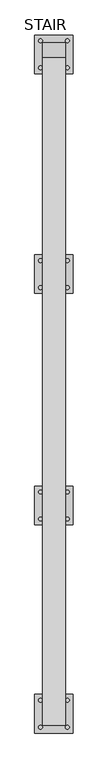
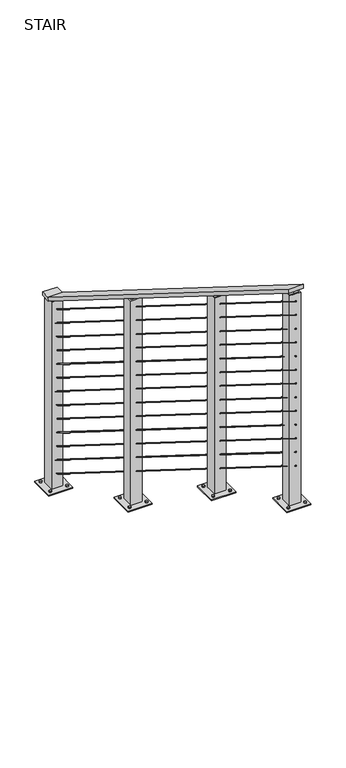
"""IFC4 building model written with IfcOpenShell, lengths in millimetres: railing geometry, STAIR."""

from ifc_helpers import new_model, si_unit, point, frame, frame_2d, origin, origin_with_axes, place, context, project, spatial, polyline, circle_curve, ellipse_curve, trimmed, segment, composite_curve, outline, extrude, faceted_brep, source, transform, mapped, element, save
from ifc_brep_helpers import plane_surface, cylinder_surface, advanced_brep


def stair_e71d8709(model_context):
    return source(origin(), model_context, "Body", "SolidModel", [
        faceted_brep([(27258.1620052, 6154.2043237, 1066.8), (27334.3620052, 6154.2043237, 1066.8), (27334.3620052, 6154.2043237, 1047.75), (27258.1620052, 6154.2043237, 1047.75), (27258.1620052, 6106.1413199, 1066.8), (27334.3620052, 6106.1413199, 1066.8), (27334.3620052, 6100.6673274, 1047.75), (27258.1620052, 3906.3043237, 2444.8228911), (27258.1620052, 3906.3043237, 2422.3438702), (27334.3620052, 3906.3043237, 2422.3438702), (27334.3620052, 3906.3043237, 2444.8228911), (27258.1620052, 6100.6673274, 1047.75)], [[[0, 1, 2, 3]], [[1, 0, 4, 5]], [[2, 1, 5, 6]], [[7, 8, 9, 10]], [[5, 4, 7, 10]], [[6, 5, 10, 9]], [[3, 2, 6, 11]], [[0, 3, 11, 4]], [[11, 6, 9, 8]], [[4, 11, 8, 7]]]),
        advanced_brep(
        [(27298.6432552, 6154.2043237, 988.21875), (27293.8807552, 6154.2043237, 988.21875), (27298.6432552, 3906.3043237, 2364.0985031), (27293.8807552, 3906.3043237, 2364.0985031), (27298.6432552, 6102.7200746, 988.21875), (27293.8807552, 6102.7200746, 988.21875)],
        [
            (0, 1, circle_curve(frame((27296.2620052, 6154.2043237, 988.21875), z_axis=(0.0, 1.0, 0.0), x_axis=(-1.0, 0.0, 0.0)), 2.38125)),
            (1, 0, circle_curve(frame((27296.2620052, 6154.2043237, 988.21875), z_axis=(0.0, 1.0, 0.0), x_axis=(-1.0, 0.0, 0.0)), 2.38125)),
            (2, 3, ellipse_curve(frame((27296.2620052, 3906.3043237, 2364.0985031), z_axis=(0.0, -1.0, 0.0), x_axis=(0.0, 0.0, -1.0)), 2.8098776, 2.38125)),
            (3, 2, ellipse_curve(frame((27296.2620052, 3906.3043237, 2364.0985031), z_axis=(0.0, -1.0, 0.0), x_axis=(0.0, 0.0, -1.0)), 2.8098776, 2.38125)),
            (0, 4),
            (4, 5, ellipse_curve(frame((27296.2620052, 6102.7200746, 988.21875), z_axis=(0.0, 0.9611079128273463, -0.2761730977134851), x_axis=(0.0, 0.27617309771348497, 0.9611079128273464)), 2.4776094, 2.38125)),
            (5, 1),
            (5, 4, ellipse_curve(frame((27296.2620052, 6102.7200746, 988.21875), z_axis=(0.0, 0.9611079128273463, -0.2761730977134851), x_axis=(0.0, 0.27617309771348497, 0.9611079128273464)), 2.4776094, 2.38125)),
            (4, 2),
            (3, 5),
        ],
        [
            plane_surface(frame((27296.2620052, 6154.2043237, 990.6), z_axis=(0.0, 1.0, 0.0), x_axis=(0.0, 0.0, -1.0))),
            plane_surface(frame((27296.2620052, 3906.3043237, 2366.9083807), z_axis=(0.0, -1.0, 0.0), x_axis=(0.0, 0.0, -1.0))),
            cylinder_surface(frame((27296.2620052, 6154.2043237, 988.21875), z_axis=(0.0, 1.0, 0.0), x_axis=(-1.0, 0.0, 0.0)), 2.38125),
            cylinder_surface(frame((27296.2620052, 6102.1402031, 988.5819934), z_axis=(0.0, 0.8474568401986756, -0.5308642990449408), x_axis=(-1.0, 0.0, 0.0)), 2.38125),
        ],
        [
            (0, [[1, 2]]),
            (1, [[3, 4]]),
            (2, [[-1, 5, 6, 7]]),
            (2, [[-2, -7, 8, -5]]),
            (3, [[-6, 9, -4, 10]]),
            (3, [[-8, -10, -3, -9]]),
        ],
    ),
        advanced_brep(
        [(27298.6432552, 6154.2043237, 912.01875), (27293.8807552, 6154.2043237, 912.01875), (27298.6432552, 6102.7200746, 912.01875), (27293.8807552, 6102.7200746, 912.01875), (27298.6432552, 3906.3043237, 2287.8985031), (27293.8807552, 3906.3043237, 2287.8985031)],
        [
            (0, 1, circle_curve(frame((27296.2620052, 6154.2043237, 912.01875), z_axis=(0.0, 1.0, 0.0), x_axis=(-1.0, 0.0, 0.0)), 2.38125)),
            (1, 0, circle_curve(frame((27296.2620052, 6154.2043237, 912.01875), z_axis=(0.0, 1.0, 0.0), x_axis=(-1.0, 0.0, 0.0)), 2.38125)),
            (0, 2),
            (2, 3, ellipse_curve(frame((27296.2620052, 6102.7200746, 912.01875), z_axis=(0.0, 0.9611079128273463, -0.2761730977134851), x_axis=(0.0, 0.27617309771348497, 0.9611079128273464)), 2.4776094, 2.38125)),
            (3, 1),
            (3, 2, ellipse_curve(frame((27296.2620052, 6102.7200746, 912.01875), z_axis=(0.0, 0.9611079128273463, -0.2761730977134851), x_axis=(0.0, 0.27617309771348497, 0.9611079128273464)), 2.4776094, 2.38125)),
            (4, 5, ellipse_curve(frame((27296.2620052, 3906.3043237, 2287.8985031), z_axis=(0.0, -1.0, 0.0), x_axis=(0.0, 0.0, -1.0)), 2.8098776, 2.38125)),
            (5, 4, ellipse_curve(frame((27296.2620052, 3906.3043237, 2287.8985031), z_axis=(0.0, -1.0, 0.0), x_axis=(0.0, 0.0, -1.0)), 2.8098776, 2.38125)),
            (2, 4),
            (5, 3),
        ],
        [
            plane_surface(frame((27296.2620052, 6154.2043237, 914.4), z_axis=(0.0, 1.0, 0.0), x_axis=(0.0, 0.0, -1.0))),
            cylinder_surface(frame((27296.2620052, 6154.2043237, 912.01875), z_axis=(0.0, 1.0, 0.0), x_axis=(-1.0, 0.0, 0.0)), 2.38125),
            plane_surface(frame((27296.2620052, 3906.3043237, 2290.7083807), z_axis=(0.0, -1.0, 0.0), x_axis=(0.0, 0.0, -1.0))),
            cylinder_surface(frame((27296.2620052, 6102.1402031, 912.3819934), z_axis=(0.0, 0.8474568401986756, -0.5308642990449408), x_axis=(-1.0, 0.0, 0.0)), 2.38125),
        ],
        [
            (0, [[1, 2]]),
            (1, [[-1, 3, 4, 5]]),
            (1, [[-2, -5, 6, -3]]),
            (2, [[7, 8]]),
            (3, [[-4, 9, -8, 10]]),
            (3, [[-6, -10, -7, -9]]),
        ],
    ),
        advanced_brep(
        [(27298.6432552, 6154.2043237, 835.81875), (27293.8807552, 6154.2043237, 835.81875), (27298.6432552, 6102.7200746, 835.81875), (27293.8807552, 6102.7200746, 835.81875), (27298.6432552, 3906.3043237, 2211.6985031), (27293.8807552, 3906.3043237, 2211.6985031)],
        [
            (0, 1, circle_curve(frame((27296.2620052, 6154.2043237, 835.81875), z_axis=(0.0, 1.0, 0.0), x_axis=(-1.0, 0.0, 0.0)), 2.38125)),
            (1, 0, circle_curve(frame((27296.2620052, 6154.2043237, 835.81875), z_axis=(0.0, 1.0, 0.0), x_axis=(-1.0, 0.0, 0.0)), 2.38125)),
            (0, 2),
            (2, 3, ellipse_curve(frame((27296.2620052, 6102.7200746, 835.81875), z_axis=(0.0, 0.9611079128273463, -0.2761730977134851), x_axis=(0.0, 0.27617309771348497, 0.9611079128273464)), 2.4776094, 2.38125)),
            (3, 1),
            (3, 2, ellipse_curve(frame((27296.2620052, 6102.7200746, 835.81875), z_axis=(0.0, 0.9611079128273463, -0.2761730977134851), x_axis=(0.0, 0.27617309771348497, 0.9611079128273464)), 2.4776094, 2.38125)),
            (4, 5, ellipse_curve(frame((27296.2620052, 3906.3043237, 2211.6985031), z_axis=(0.0, -1.0, 0.0), x_axis=(0.0, 0.0, -1.0)), 2.8098776, 2.38125)),
            (5, 4, ellipse_curve(frame((27296.2620052, 3906.3043237, 2211.6985031), z_axis=(0.0, -1.0, 0.0), x_axis=(0.0, 0.0, -1.0)), 2.8098776, 2.38125)),
            (2, 4),
            (5, 3),
        ],
        [
            plane_surface(frame((27296.2620052, 6154.2043237, 838.2), z_axis=(0.0, 1.0, 0.0), x_axis=(0.0, 0.0, -1.0))),
            cylinder_surface(frame((27296.2620052, 6154.2043237, 835.81875), z_axis=(0.0, 1.0, 0.0), x_axis=(-1.0, 0.0, 0.0)), 2.38125),
            plane_surface(frame((27296.2620052, 3906.3043237, 2214.5083807), z_axis=(0.0, -1.0, 0.0), x_axis=(0.0, 0.0, -1.0))),
            cylinder_surface(frame((27296.2620052, 6102.1402031, 836.1819934), z_axis=(0.0, 0.8474568401986756, -0.5308642990449408), x_axis=(-1.0, 0.0, 0.0)), 2.38125),
        ],
        [
            (0, [[1, 2]]),
            (1, [[-1, 3, 4, 5]]),
            (1, [[-2, -5, 6, -3]]),
            (2, [[7, 8]]),
            (3, [[-4, 9, -8, 10]]),
            (3, [[-6, -10, -7, -9]]),
        ],
    ),
        advanced_brep(
        [(27298.6432552, 6154.2043237, 759.61875), (27293.8807552, 6154.2043237, 759.61875), (27298.6432552, 6102.7200746, 759.61875), (27293.8807552, 6102.7200746, 759.61875), (27298.6432552, 3906.3043237, 2135.4985031), (27293.8807552, 3906.3043237, 2135.4985031)],
        [
            (0, 1, circle_curve(frame((27296.2620052, 6154.2043237, 759.61875), z_axis=(0.0, 1.0, 0.0), x_axis=(-1.0, 0.0, 0.0)), 2.38125)),
            (1, 0, circle_curve(frame((27296.2620052, 6154.2043237, 759.61875), z_axis=(0.0, 1.0, 0.0), x_axis=(-1.0, 0.0, 0.0)), 2.38125)),
            (0, 2),
            (2, 3, ellipse_curve(frame((27296.2620052, 6102.7200746, 759.61875), z_axis=(0.0, 0.9611079128273463, -0.2761730977134851), x_axis=(0.0, 0.27617309771348497, 0.9611079128273464)), 2.4776094, 2.38125)),
            (3, 1),
            (3, 2, ellipse_curve(frame((27296.2620052, 6102.7200746, 759.61875), z_axis=(0.0, 0.9611079128273463, -0.2761730977134851), x_axis=(0.0, 0.27617309771348497, 0.9611079128273464)), 2.4776094, 2.38125)),
            (4, 5, ellipse_curve(frame((27296.2620052, 3906.3043237, 2135.4985031), z_axis=(0.0, -1.0, 0.0), x_axis=(0.0, 0.0, -1.0)), 2.8098776, 2.38125)),
            (5, 4, ellipse_curve(frame((27296.2620052, 3906.3043237, 2135.4985031), z_axis=(0.0, -1.0, 0.0), x_axis=(0.0, 0.0, -1.0)), 2.8098776, 2.38125)),
            (2, 4),
            (5, 3),
        ],
        [
            plane_surface(frame((27296.2620052, 6154.2043237, 762.0), z_axis=(0.0, 1.0, 0.0), x_axis=(0.0, 0.0, -1.0))),
            cylinder_surface(frame((27296.2620052, 6154.2043237, 759.61875), z_axis=(0.0, 1.0, 0.0), x_axis=(-1.0, 0.0, 0.0)), 2.38125),
            plane_surface(frame((27296.2620052, 3906.3043237, 2138.3083807), z_axis=(0.0, -1.0, 0.0), x_axis=(0.0, 0.0, -1.0))),
            cylinder_surface(frame((27296.2620052, 6102.1402031, 759.9819934), z_axis=(0.0, 0.8474568401986756, -0.5308642990449408), x_axis=(-1.0, 0.0, 0.0)), 2.38125),
        ],
        [
            (0, [[1, 2]]),
            (1, [[-1, 3, 4, 5]]),
            (1, [[-2, -5, 6, -3]]),
            (2, [[7, 8]]),
            (3, [[-4, 9, -8, 10]]),
            (3, [[-6, -10, -7, -9]]),
        ],
    ),
        advanced_brep(
        [(27298.6432552, 6154.2043237, 683.41875), (27293.8807552, 6154.2043237, 683.41875), (27298.6432552, 6102.7200746, 683.41875), (27293.8807552, 6102.7200746, 683.41875), (27298.6432552, 3906.3043237, 2059.2985031), (27293.8807552, 3906.3043237, 2059.2985031)],
        [
            (0, 1, circle_curve(frame((27296.2620052, 6154.2043237, 683.41875), z_axis=(0.0, 1.0, 0.0), x_axis=(-1.0, 0.0, 0.0)), 2.38125)),
            (1, 0, circle_curve(frame((27296.2620052, 6154.2043237, 683.41875), z_axis=(0.0, 1.0, 0.0), x_axis=(-1.0, 0.0, 0.0)), 2.38125)),
            (0, 2),
            (2, 3, ellipse_curve(frame((27296.2620052, 6102.7200746, 683.41875), z_axis=(0.0, 0.9611079128273463, -0.2761730977134851), x_axis=(0.0, 0.27617309771348497, 0.9611079128273464)), 2.4776094, 2.38125)),
            (3, 1),
            (3, 2, ellipse_curve(frame((27296.2620052, 6102.7200746, 683.41875), z_axis=(0.0, 0.9611079128273463, -0.2761730977134851), x_axis=(0.0, 0.27617309771348497, 0.9611079128273464)), 2.4776094, 2.38125)),
            (4, 5, ellipse_curve(frame((27296.2620052, 3906.3043237, 2059.2985031), z_axis=(0.0, -1.0, 0.0), x_axis=(0.0, 0.0, -1.0)), 2.8098776, 2.38125)),
            (5, 4, ellipse_curve(frame((27296.2620052, 3906.3043237, 2059.2985031), z_axis=(0.0, -1.0, 0.0), x_axis=(0.0, 0.0, -1.0)), 2.8098776, 2.38125)),
            (2, 4),
            (5, 3),
        ],
        [
            plane_surface(frame((27296.2620052, 6154.2043237, 685.8), z_axis=(0.0, 1.0, 0.0), x_axis=(0.0, 0.0, -1.0))),
            cylinder_surface(frame((27296.2620052, 6154.2043237, 683.41875), z_axis=(0.0, 1.0, 0.0), x_axis=(-1.0, 0.0, 0.0)), 2.38125),
            plane_surface(frame((27296.2620052, 3906.3043237, 2062.1083807), z_axis=(0.0, -1.0, 0.0), x_axis=(0.0, 0.0, -1.0))),
            cylinder_surface(frame((27296.2620052, 6102.1402031, 683.7819934), z_axis=(0.0, 0.8474568401986756, -0.5308642990449408), x_axis=(-1.0, 0.0, 0.0)), 2.38125),
        ],
        [
            (0, [[1, 2]]),
            (1, [[-1, 3, 4, 5]]),
            (1, [[-2, -5, 6, -3]]),
            (2, [[7, 8]]),
            (3, [[-4, 9, -8, 10]]),
            (3, [[-6, -10, -7, -9]]),
        ],
    ),
        advanced_brep(
        [(27298.6432552, 6154.2043237, 607.21875), (27293.8807552, 6154.2043237, 607.21875), (27298.6432552, 6102.7200746, 607.21875), (27293.8807552, 6102.7200746, 607.21875), (27298.6432552, 3906.3043237, 1983.0985031), (27293.8807552, 3906.3043237, 1983.0985031)],
        [
            (0, 1, circle_curve(frame((27296.2620052, 6154.2043237, 607.21875), z_axis=(0.0, 1.0, 0.0), x_axis=(-1.0, 0.0, 0.0)), 2.38125)),
            (1, 0, circle_curve(frame((27296.2620052, 6154.2043237, 607.21875), z_axis=(0.0, 1.0, 0.0), x_axis=(-1.0, 0.0, 0.0)), 2.38125)),
            (0, 2),
            (2, 3, ellipse_curve(frame((27296.2620052, 6102.7200746, 607.21875), z_axis=(0.0, 0.9611079128273463, -0.2761730977134851), x_axis=(0.0, 0.27617309771348497, 0.9611079128273464)), 2.4776094, 2.38125)),
            (3, 1),
            (3, 2, ellipse_curve(frame((27296.2620052, 6102.7200746, 607.21875), z_axis=(0.0, 0.9611079128273463, -0.2761730977134851), x_axis=(0.0, 0.27617309771348497, 0.9611079128273464)), 2.4776094, 2.38125)),
            (4, 5, ellipse_curve(frame((27296.2620052, 3906.3043237, 1983.0985031), z_axis=(0.0, -1.0, 0.0), x_axis=(0.0, 0.0, -1.0)), 2.8098776, 2.38125)),
            (5, 4, ellipse_curve(frame((27296.2620052, 3906.3043237, 1983.0985031), z_axis=(0.0, -1.0, 0.0), x_axis=(0.0, 0.0, -1.0)), 2.8098776, 2.38125)),
            (2, 4),
            (5, 3),
        ],
        [
            plane_surface(frame((27296.2620052, 6154.2043237, 609.6), z_axis=(0.0, 1.0, 0.0), x_axis=(0.0, 0.0, -1.0))),
            cylinder_surface(frame((27296.2620052, 6154.2043237, 607.21875), z_axis=(0.0, 1.0, 0.0), x_axis=(-1.0, 0.0, 0.0)), 2.38125),
            plane_surface(frame((27296.2620052, 3906.3043237, 1985.9083807), z_axis=(0.0, -1.0, 0.0), x_axis=(0.0, 0.0, -1.0))),
            cylinder_surface(frame((27296.2620052, 6102.1402031, 607.5819934), z_axis=(0.0, 0.8474568401986756, -0.5308642990449408), x_axis=(-1.0, 0.0, 0.0)), 2.38125),
        ],
        [
            (0, [[1, 2]]),
            (1, [[-1, 3, 4, 5]]),
            (1, [[-2, -5, 6, -3]]),
            (2, [[7, 8]]),
            (3, [[-4, 9, -8, 10]]),
            (3, [[-6, -10, -7, -9]]),
        ],
    ),
        advanced_brep(
        [(27298.6432552, 6154.2043237, 531.01875), (27293.8807552, 6154.2043237, 531.01875), (27298.6432552, 6102.7200746, 531.01875), (27293.8807552, 6102.7200746, 531.01875), (27298.6432552, 3906.3043237, 1906.8985031), (27293.8807552, 3906.3043237, 1906.8985031)],
        [
            (0, 1, circle_curve(frame((27296.2620052, 6154.2043237, 531.01875), z_axis=(0.0, 1.0, 0.0), x_axis=(-1.0, 0.0, 0.0)), 2.38125)),
            (1, 0, circle_curve(frame((27296.2620052, 6154.2043237, 531.01875), z_axis=(0.0, 1.0, 0.0), x_axis=(-1.0, 0.0, 0.0)), 2.38125)),
            (0, 2),
            (2, 3, ellipse_curve(frame((27296.2620052, 6102.7200746, 531.01875), z_axis=(0.0, 0.9611079128273463, -0.2761730977134851), x_axis=(0.0, 0.27617309771348497, 0.9611079128273464)), 2.4776094, 2.38125)),
            (3, 1),
            (3, 2, ellipse_curve(frame((27296.2620052, 6102.7200746, 531.01875), z_axis=(0.0, 0.9611079128273463, -0.2761730977134851), x_axis=(0.0, 0.27617309771348497, 0.9611079128273464)), 2.4776094, 2.38125)),
            (4, 5, ellipse_curve(frame((27296.2620052, 3906.3043237, 1906.8985031), z_axis=(0.0, -1.0, 0.0), x_axis=(0.0, 0.0, -1.0)), 2.8098776, 2.38125)),
            (5, 4, ellipse_curve(frame((27296.2620052, 3906.3043237, 1906.8985031), z_axis=(0.0, -1.0, 0.0), x_axis=(0.0, 0.0, -1.0)), 2.8098776, 2.38125)),
            (2, 4),
            (5, 3),
        ],
        [
            plane_surface(frame((27296.2620052, 6154.2043237, 533.4), z_axis=(0.0, 1.0, 0.0), x_axis=(0.0, 0.0, -1.0))),
            cylinder_surface(frame((27296.2620052, 6154.2043237, 531.01875), z_axis=(0.0, 1.0, 0.0), x_axis=(-1.0, 0.0, 0.0)), 2.38125),
            plane_surface(frame((27296.2620052, 3906.3043237, 1909.7083807), z_axis=(0.0, -1.0, 0.0), x_axis=(0.0, 0.0, -1.0))),
            cylinder_surface(frame((27296.2620052, 6102.1402031, 531.3819934), z_axis=(0.0, 0.8474568401986756, -0.5308642990449408), x_axis=(-1.0, 0.0, 0.0)), 2.38125),
        ],
        [
            (0, [[1, 2]]),
            (1, [[-1, 3, 4, 5]]),
            (1, [[-2, -5, 6, -3]]),
            (2, [[7, 8]]),
            (3, [[-4, 9, -8, 10]]),
            (3, [[-6, -10, -7, -9]]),
        ],
    ),
        advanced_brep(
        [(27298.6432552, 6154.2043237, 454.81875), (27293.8807552, 6154.2043237, 454.81875), (27298.6432552, 6102.7200746, 454.81875), (27293.8807552, 6102.7200746, 454.81875), (27298.6432552, 3906.3043237, 1830.6985031), (27293.8807552, 3906.3043237, 1830.6985031)],
        [
            (0, 1, circle_curve(frame((27296.2620052, 6154.2043237, 454.81875), z_axis=(0.0, 1.0, 0.0), x_axis=(-1.0, 0.0, 0.0)), 2.38125)),
            (1, 0, circle_curve(frame((27296.2620052, 6154.2043237, 454.81875), z_axis=(0.0, 1.0, 0.0), x_axis=(-1.0, 0.0, 0.0)), 2.38125)),
            (0, 2),
            (2, 3, ellipse_curve(frame((27296.2620052, 6102.7200746, 454.81875), z_axis=(0.0, 0.9611079128273463, -0.2761730977134851), x_axis=(0.0, 0.27617309771348497, 0.9611079128273464)), 2.4776094, 2.38125)),
            (3, 1),
            (3, 2, ellipse_curve(frame((27296.2620052, 6102.7200746, 454.81875), z_axis=(0.0, 0.9611079128273463, -0.2761730977134851), x_axis=(0.0, 0.27617309771348497, 0.9611079128273464)), 2.4776094, 2.38125)),
            (4, 5, ellipse_curve(frame((27296.2620052, 3906.3043237, 1830.6985031), z_axis=(0.0, -1.0, 0.0), x_axis=(0.0, 0.0, -1.0)), 2.8098776, 2.38125)),
            (5, 4, ellipse_curve(frame((27296.2620052, 3906.3043237, 1830.6985031), z_axis=(0.0, -1.0, 0.0), x_axis=(0.0, 0.0, -1.0)), 2.8098776, 2.38125)),
            (2, 4),
            (5, 3),
        ],
        [
            plane_surface(frame((27296.2620052, 6154.2043237, 457.2), z_axis=(0.0, 1.0, 0.0), x_axis=(0.0, 0.0, -1.0))),
            cylinder_surface(frame((27296.2620052, 6154.2043237, 454.81875), z_axis=(0.0, 1.0, 0.0), x_axis=(-1.0, 0.0, 0.0)), 2.38125),
            plane_surface(frame((27296.2620052, 3906.3043237, 1833.5083807), z_axis=(0.0, -1.0, 0.0), x_axis=(0.0, 0.0, -1.0))),
            cylinder_surface(frame((27296.2620052, 6102.1402031, 455.1819934), z_axis=(0.0, 0.8474568401986756, -0.5308642990449408), x_axis=(-1.0, 0.0, 0.0)), 2.38125),
        ],
        [
            (0, [[1, 2]]),
            (1, [[-1, 3, 4, 5]]),
            (1, [[-2, -5, 6, -3]]),
            (2, [[7, 8]]),
            (3, [[-4, 9, -8, 10]]),
            (3, [[-6, -10, -7, -9]]),
        ],
    ),
        advanced_brep(
        [(27298.6432552, 6154.2043237, 378.61875), (27293.8807552, 6154.2043237, 378.61875), (27298.6432552, 6102.7200746, 378.61875), (27293.8807552, 6102.7200746, 378.61875), (27298.6432552, 3906.3043237, 1754.4985031), (27293.8807552, 3906.3043237, 1754.4985031)],
        [
            (0, 1, circle_curve(frame((27296.2620052, 6154.2043237, 378.61875), z_axis=(0.0, 1.0, 0.0), x_axis=(-1.0, 0.0, 0.0)), 2.38125)),
            (1, 0, circle_curve(frame((27296.2620052, 6154.2043237, 378.61875), z_axis=(0.0, 1.0, 0.0), x_axis=(-1.0, 0.0, 0.0)), 2.38125)),
            (0, 2),
            (2, 3, ellipse_curve(frame((27296.2620052, 6102.7200746, 378.61875), z_axis=(0.0, 0.9611079128273463, -0.2761730977134851), x_axis=(0.0, 0.27617309771348497, 0.9611079128273464)), 2.4776094, 2.38125)),
            (3, 1),
            (3, 2, ellipse_curve(frame((27296.2620052, 6102.7200746, 378.61875), z_axis=(0.0, 0.9611079128273463, -0.2761730977134851), x_axis=(0.0, 0.27617309771348497, 0.9611079128273464)), 2.4776094, 2.38125)),
            (4, 5, ellipse_curve(frame((27296.2620052, 3906.3043237, 1754.4985031), z_axis=(0.0, -1.0, 0.0), x_axis=(0.0, 0.0, -1.0)), 2.8098776, 2.38125)),
            (5, 4, ellipse_curve(frame((27296.2620052, 3906.3043237, 1754.4985031), z_axis=(0.0, -1.0, 0.0), x_axis=(0.0, 0.0, -1.0)), 2.8098776, 2.38125)),
            (2, 4),
            (5, 3),
        ],
        [
            plane_surface(frame((27296.2620052, 6154.2043237, 381.0), z_axis=(0.0, 1.0, 0.0), x_axis=(0.0, 0.0, -1.0))),
            cylinder_surface(frame((27296.2620052, 6154.2043237, 378.61875), z_axis=(0.0, 1.0, 0.0), x_axis=(-1.0, 0.0, 0.0)), 2.38125),
            plane_surface(frame((27296.2620052, 3906.3043237, 1757.3083807), z_axis=(0.0, -1.0, 0.0), x_axis=(0.0, 0.0, -1.0))),
            cylinder_surface(frame((27296.2620052, 6102.1402031, 378.9819934), z_axis=(0.0, 0.8474568401986756, -0.5308642990449408), x_axis=(-1.0, 0.0, 0.0)), 2.38125),
        ],
        [
            (0, [[1, 2]]),
            (1, [[-1, 3, 4, 5]]),
            (1, [[-2, -5, 6, -3]]),
            (2, [[7, 8]]),
            (3, [[-4, 9, -8, 10]]),
            (3, [[-6, -10, -7, -9]]),
        ],
    ),
        advanced_brep(
        [(27298.6432552, 6154.2043237, 302.41875), (27293.8807552, 6154.2043237, 302.41875), (27298.6432552, 6102.7200746, 302.41875), (27293.8807552, 6102.7200746, 302.41875), (27298.6432552, 3906.3043237, 1678.2985031), (27293.8807552, 3906.3043237, 1678.2985031)],
        [
            (0, 1, circle_curve(frame((27296.2620052, 6154.2043237, 302.41875), z_axis=(0.0, 1.0, 0.0), x_axis=(-1.0, 0.0, 0.0)), 2.38125)),
            (1, 0, circle_curve(frame((27296.2620052, 6154.2043237, 302.41875), z_axis=(0.0, 1.0, 0.0), x_axis=(-1.0, 0.0, 0.0)), 2.38125)),
            (0, 2),
            (2, 3, ellipse_curve(frame((27296.2620052, 6102.7200746, 302.41875), z_axis=(0.0, 0.9611079128273463, -0.2761730977134851), x_axis=(0.0, 0.27617309771348497, 0.9611079128273464)), 2.4776094, 2.38125)),
            (3, 1),
            (3, 2, ellipse_curve(frame((27296.2620052, 6102.7200746, 302.41875), z_axis=(0.0, 0.9611079128273463, -0.2761730977134851), x_axis=(0.0, 0.27617309771348497, 0.9611079128273464)), 2.4776094, 2.38125)),
            (4, 5, ellipse_curve(frame((27296.2620052, 3906.3043237, 1678.2985031), z_axis=(0.0, -1.0, 0.0), x_axis=(0.0, 0.0, -1.0)), 2.8098776, 2.38125)),
            (5, 4, ellipse_curve(frame((27296.2620052, 3906.3043237, 1678.2985031), z_axis=(0.0, -1.0, 0.0), x_axis=(0.0, 0.0, -1.0)), 2.8098776, 2.38125)),
            (2, 4),
            (5, 3),
        ],
        [
            plane_surface(frame((27296.2620052, 6154.2043237, 304.8), z_axis=(0.0, 1.0, 0.0), x_axis=(0.0, 0.0, -1.0))),
            cylinder_surface(frame((27296.2620052, 6154.2043237, 302.41875), z_axis=(0.0, 1.0, 0.0), x_axis=(-1.0, 0.0, 0.0)), 2.38125),
            plane_surface(frame((27296.2620052, 3906.3043237, 1681.1083807), z_axis=(0.0, -1.0, 0.0), x_axis=(0.0, 0.0, -1.0))),
            cylinder_surface(frame((27296.2620052, 6102.1402031, 302.7819934), z_axis=(0.0, 0.8474568401986756, -0.5308642990449408), x_axis=(-1.0, 0.0, 0.0)), 2.38125),
        ],
        [
            (0, [[1, 2]]),
            (1, [[-1, 3, 4, 5]]),
            (1, [[-2, -5, 6, -3]]),
            (2, [[7, 8]]),
            (3, [[-4, 9, -8, 10]]),
            (3, [[-6, -10, -7, -9]]),
        ],
    ),
        advanced_brep(
        [(27298.6432552, 6154.2043237, 226.21875), (27293.8807552, 6154.2043237, 226.21875), (27298.6432552, 6102.7200746, 226.21875), (27293.8807552, 6102.7200746, 226.21875), (27298.6432552, 3906.3043237, 1602.0985031), (27293.8807552, 3906.3043237, 1602.0985031)],
        [
            (0, 1, circle_curve(frame((27296.2620052, 6154.2043237, 226.21875), z_axis=(0.0, 1.0, 0.0), x_axis=(-1.0, 0.0, 0.0)), 2.38125)),
            (1, 0, circle_curve(frame((27296.2620052, 6154.2043237, 226.21875), z_axis=(0.0, 1.0, 0.0), x_axis=(-1.0, 0.0, 0.0)), 2.38125)),
            (0, 2),
            (2, 3, ellipse_curve(frame((27296.2620052, 6102.7200746, 226.21875), z_axis=(0.0, 0.9611079128273463, -0.2761730977134851), x_axis=(0.0, 0.27617309771348497, 0.9611079128273464)), 2.4776094, 2.38125)),
            (3, 1),
            (3, 2, ellipse_curve(frame((27296.2620052, 6102.7200746, 226.21875), z_axis=(0.0, 0.9611079128273463, -0.2761730977134851), x_axis=(0.0, 0.27617309771348497, 0.9611079128273464)), 2.4776094, 2.38125)),
            (4, 5, ellipse_curve(frame((27296.2620052, 3906.3043237, 1602.0985031), z_axis=(0.0, -1.0, 0.0), x_axis=(0.0, 0.0, -1.0)), 2.8098776, 2.38125)),
            (5, 4, ellipse_curve(frame((27296.2620052, 3906.3043237, 1602.0985031), z_axis=(0.0, -1.0, 0.0), x_axis=(0.0, 0.0, -1.0)), 2.8098776, 2.38125)),
            (2, 4),
            (5, 3),
        ],
        [
            plane_surface(frame((27296.2620052, 6154.2043237, 228.6), z_axis=(0.0, 1.0, 0.0), x_axis=(0.0, 0.0, -1.0))),
            cylinder_surface(frame((27296.2620052, 6154.2043237, 226.21875), z_axis=(0.0, 1.0, 0.0), x_axis=(-1.0, 0.0, 0.0)), 2.38125),
            plane_surface(frame((27296.2620052, 3906.3043237, 1604.9083807), z_axis=(0.0, -1.0, 0.0), x_axis=(0.0, 0.0, -1.0))),
            cylinder_surface(frame((27296.2620052, 6102.1402031, 226.5819934), z_axis=(0.0, 0.8474568401986756, -0.5308642990449408), x_axis=(-1.0, 0.0, 0.0)), 2.38125),
        ],
        [
            (0, [[1, 2]]),
            (1, [[-1, 3, 4, 5]]),
            (1, [[-2, -5, 6, -3]]),
            (2, [[7, 8]]),
            (3, [[-4, 9, -8, 10]]),
            (3, [[-6, -10, -7, -9]]),
        ],
    ),
        advanced_brep(
        [(27298.6432552, 6154.2043237, 150.01875), (27293.8807552, 6154.2043237, 150.01875), (27298.6432552, 6102.7200746, 150.01875), (27293.8807552, 6102.7200746, 150.01875), (27298.6432552, 3906.3043237, 1525.8985031), (27293.8807552, 3906.3043237, 1525.8985031)],
        [
            (0, 1, circle_curve(frame((27296.2620052, 6154.2043237, 150.01875), z_axis=(0.0, 1.0, 0.0), x_axis=(-1.0, 0.0, 0.0)), 2.38125)),
            (1, 0, circle_curve(frame((27296.2620052, 6154.2043237, 150.01875), z_axis=(0.0, 1.0, 0.0), x_axis=(-1.0, 0.0, 0.0)), 2.38125)),
            (0, 2),
            (2, 3, ellipse_curve(frame((27296.2620052, 6102.7200746, 150.01875), z_axis=(0.0, 0.9611079128273463, -0.2761730977134851), x_axis=(0.0, 0.27617309771348497, 0.9611079128273464)), 2.4776094, 2.38125)),
            (3, 1),
            (3, 2, ellipse_curve(frame((27296.2620052, 6102.7200746, 150.01875), z_axis=(0.0, 0.9611079128273463, -0.2761730977134851), x_axis=(0.0, 0.27617309771348497, 0.9611079128273464)), 2.4776094, 2.38125)),
            (4, 5, ellipse_curve(frame((27296.2620052, 3906.3043237, 1525.8985031), z_axis=(0.0, -1.0, 0.0), x_axis=(0.0, 0.0, -1.0)), 2.8098776, 2.38125)),
            (5, 4, ellipse_curve(frame((27296.2620052, 3906.3043237, 1525.8985031), z_axis=(0.0, -1.0, 0.0), x_axis=(0.0, 0.0, -1.0)), 2.8098776, 2.38125)),
            (2, 4),
            (5, 3),
        ],
        [
            plane_surface(frame((27296.2620052, 6154.2043237, 152.4), z_axis=(0.0, 1.0, 0.0), x_axis=(0.0, 0.0, -1.0))),
            cylinder_surface(frame((27296.2620052, 6154.2043237, 150.01875), z_axis=(0.0, 1.0, 0.0), x_axis=(-1.0, 0.0, 0.0)), 2.38125),
            plane_surface(frame((27296.2620052, 3906.3043237, 1528.7083807), z_axis=(0.0, -1.0, 0.0), x_axis=(0.0, 0.0, -1.0))),
            cylinder_surface(frame((27296.2620052, 6102.1402031, 150.3819934), z_axis=(0.0, 0.8474568401986756, -0.5308642990449408), x_axis=(-1.0, 0.0, 0.0)), 2.38125),
        ],
        [
            (0, [[1, 2]]),
            (1, [[-1, 3, 4, 5]]),
            (1, [[-2, -5, 6, -3]]),
            (2, [[7, 8]]),
            (3, [[-4, 9, -8, 10]]),
            (3, [[-6, -10, -7, -9]]),
        ],
    ),
        advanced_brep(
        [(27298.6432552, 6154.2043237, 73.81875), (27293.8807552, 6154.2043237, 73.81875), (27298.6432552, 6102.7200746, 73.81875), (27293.8807552, 6102.7200746, 73.81875), (27298.6432552, 3906.3043237, 1449.6985031), (27293.8807552, 3906.3043237, 1449.6985031)],
        [
            (0, 1, circle_curve(frame((27296.2620052, 6154.2043237, 73.81875), z_axis=(0.0, 1.0, 0.0), x_axis=(-1.0, 0.0, 0.0)), 2.38125)),
            (1, 0, circle_curve(frame((27296.2620052, 6154.2043237, 73.81875), z_axis=(0.0, 1.0, 0.0), x_axis=(-1.0, 0.0, 0.0)), 2.38125)),
            (0, 2),
            (2, 3, ellipse_curve(frame((27296.2620052, 6102.7200746, 73.81875), z_axis=(0.0, 0.9611079128273463, -0.2761730977134851), x_axis=(0.0, 0.27617309771348497, 0.9611079128273464)), 2.4776094, 2.38125)),
            (3, 1),
            (3, 2, ellipse_curve(frame((27296.2620052, 6102.7200746, 73.81875), z_axis=(0.0, 0.9611079128273463, -0.2761730977134851), x_axis=(0.0, 0.27617309771348497, 0.9611079128273464)), 2.4776094, 2.38125)),
            (4, 5, ellipse_curve(frame((27296.2620052, 3906.3043237, 1449.6985031), z_axis=(0.0, -1.0, 0.0), x_axis=(0.0, 0.0, -1.0)), 2.8098776, 2.38125)),
            (5, 4, ellipse_curve(frame((27296.2620052, 3906.3043237, 1449.6985031), z_axis=(0.0, -1.0, 0.0), x_axis=(0.0, 0.0, -1.0)), 2.8098776, 2.38125)),
            (2, 4),
            (5, 3),
        ],
        [
            plane_surface(frame((27296.2620052, 6154.2043237, 76.2), z_axis=(0.0, 1.0, 0.0), x_axis=(0.0, 0.0, -1.0))),
            cylinder_surface(frame((27296.2620052, 6154.2043237, 73.81875), z_axis=(0.0, 1.0, 0.0), x_axis=(-1.0, 0.0, 0.0)), 2.38125),
            plane_surface(frame((27296.2620052, 3906.3043237, 1452.5083807), z_axis=(0.0, -1.0, 0.0), x_axis=(0.0, 0.0, -1.0))),
            cylinder_surface(frame((27296.2620052, 6102.1402031, 74.1819934), z_axis=(0.0, 0.8474568401986756, -0.5308642990449408), x_axis=(-1.0, 0.0, 0.0)), 2.38125),
        ],
        [
            (0, [[1, 2]]),
            (1, [[-1, 3, 4, 5]]),
            (1, [[-2, -5, 6, -3]]),
            (2, [[7, 8]]),
            (3, [[-4, 9, -8, 10]]),
            (3, [[-6, -10, -7, -9]]),
        ],
    ),
        extrude(outline(composite_curve([segment(trimmed(circle_curve(frame_2d((27251.8120052, 4674.6543237)), 6.35), [point((27245.4620052, 4674.6543237))], [point((27258.1620052, 4674.6543237))], False, "CARTESIAN"), True, "CONTINUOUS"), segment(trimmed(circle_curve(frame_2d((27251.8120052, 4674.6543237)), 6.35), [point((27258.1620052, 4674.6543237))], [point((27245.4620052, 4674.6543237))], False, "CARTESIAN"), True, "CONTINUOUS")], self_intersect=False)), frame((0.0, 0.0, 875.109375), z_axis=(0.0, 0.0, 1.0), x_axis=(1.0, 0.0, 0.0)), (0.0, 0.0, 1.0), 12.7),
        extrude(outline(composite_curve([segment(trimmed(circle_curve(frame_2d((27340.7120052, 4674.6543237)), 6.35), [point((27334.3620052, 4674.6543237))], [point((27347.0620052, 4674.6543237))], False, "CARTESIAN"), True, "CONTINUOUS"), segment(trimmed(circle_curve(frame_2d((27340.7120052, 4674.6543237)), 6.35), [point((27347.0620052, 4674.6543237))], [point((27334.3620052, 4674.6543237))], False, "CARTESIAN"), True, "CONTINUOUS")], self_intersect=False)), frame((0.0, 0.0, 875.109375), z_axis=(0.0, 0.0, 1.0), x_axis=(1.0, 0.0, 0.0)), (0.0, 0.0, 1.0), 12.7),
        extrude(outline(composite_curve([segment(trimmed(circle_curve(frame_2d((27251.8120052, 4585.7543237)), 6.35), [point((27245.4620052, 4585.7543237))], [point((27258.1620052, 4585.7543237))], False, "CARTESIAN"), True, "CONTINUOUS"), segment(trimmed(circle_curve(frame_2d((27251.8120052, 4585.7543237)), 6.35), [point((27258.1620052, 4585.7543237))], [point((27245.4620052, 4585.7543237))], False, "CARTESIAN"), True, "CONTINUOUS")], self_intersect=False)), frame((0.0, 0.0, 875.109375), z_axis=(0.0, 0.0, 1.0), x_axis=(1.0, 0.0, 0.0)), (0.0, 0.0, 1.0), 12.7),
        extrude(outline(composite_curve([segment(trimmed(circle_curve(frame_2d((27340.7120052, 4585.7543237)), 6.35), [point((27334.3620052, 4585.7543237))], [point((27347.0620052, 4585.7543237))], False, "CARTESIAN"), True, "CONTINUOUS"), segment(trimmed(circle_curve(frame_2d((27340.7120052, 4585.7543237)), 6.35), [point((27347.0620052, 4585.7543237))], [point((27334.3620052, 4585.7543237))], False, "CARTESIAN"), True, "CONTINUOUS")], self_intersect=False)), frame((0.0, 0.0, 875.109375), z_axis=(0.0, 0.0, 1.0), x_axis=(1.0, 0.0, 0.0)), (0.0, 0.0, 1.0), 12.7),
        extrude(outline(polyline([(27359.7620052, 4693.7043237), (27359.7620052, 4566.7043237), (27232.7620052, 4566.7043237), (27232.7620052, 4693.7043237), (27359.7620052, 4693.7043237)])), frame((0.0, 0.0, 875.109375), z_axis=(0.0, 0.0, 1.0), x_axis=(1.0, 0.0, 0.0)), (0.0, 0.0, 1.0), 6.35),
        extrude(outline(polyline([(27326.4245052, 4660.3668237), (27326.4245052, 4600.0418237), (27266.0995052, 4600.0418237), (27266.0995052, 4660.3668237), (27326.4245052, 4660.3668237)]), holes=[polyline([(27320.0745052, 4654.0168237), (27272.4495052, 4654.0168237), (27272.4495052, 4606.3918237), (27320.0745052, 4606.3918237), (27320.0745052, 4654.0168237)])]), frame((0.0, 0.0, 875.109375), z_axis=(0.0, 0.0, 1.0), x_axis=(1.0, 0.0, 0.0)), (0.0, 0.0, 1.0), 1095.4832386),
        extrude(outline(composite_curve([segment(trimmed(circle_curve(frame_2d((27251.8120052, 5436.6543237)), 6.35), [point((27245.4620052, 5436.6543237))], [point((27258.1620052, 5436.6543237))], False, "CARTESIAN"), True, "CONTINUOUS"), segment(trimmed(circle_curve(frame_2d((27251.8120052, 5436.6543237)), 6.35), [point((27258.1620052, 5436.6543237))], [point((27245.4620052, 5436.6543237))], False, "CARTESIAN"), True, "CONTINUOUS")], self_intersect=False)), frame((0.0, 0.0, 350.04375), z_axis=(0.0, 0.0, 1.0), x_axis=(1.0, 0.0, 0.0)), (0.0, 0.0, 1.0), 12.7),
        extrude(outline(composite_curve([segment(trimmed(circle_curve(frame_2d((27340.7120052, 5436.6543237)), 6.35), [point((27334.3620052, 5436.6543237))], [point((27347.0620052, 5436.6543237))], False, "CARTESIAN"), True, "CONTINUOUS"), segment(trimmed(circle_curve(frame_2d((27340.7120052, 5436.6543237)), 6.35), [point((27347.0620052, 5436.6543237))], [point((27334.3620052, 5436.6543237))], False, "CARTESIAN"), True, "CONTINUOUS")], self_intersect=False)), frame((0.0, 0.0, 350.04375), z_axis=(0.0, 0.0, 1.0), x_axis=(1.0, 0.0, 0.0)), (0.0, 0.0, 1.0), 12.7),
        extrude(outline(composite_curve([segment(trimmed(circle_curve(frame_2d((27251.8120052, 5347.7543237)), 6.35), [point((27245.4620052, 5347.7543237))], [point((27258.1620052, 5347.7543237))], False, "CARTESIAN"), True, "CONTINUOUS"), segment(trimmed(circle_curve(frame_2d((27251.8120052, 5347.7543237)), 6.35), [point((27258.1620052, 5347.7543237))], [point((27245.4620052, 5347.7543237))], False, "CARTESIAN"), True, "CONTINUOUS")], self_intersect=False)), frame((0.0, 0.0, 350.04375), z_axis=(0.0, 0.0, 1.0), x_axis=(1.0, 0.0, 0.0)), (0.0, 0.0, 1.0), 12.7),
        extrude(outline(composite_curve([segment(trimmed(circle_curve(frame_2d((27340.7120052, 5347.7543237)), 6.35), [point((27334.3620052, 5347.7543237))], [point((27347.0620052, 5347.7543237))], False, "CARTESIAN"), True, "CONTINUOUS"), segment(trimmed(circle_curve(frame_2d((27340.7120052, 5347.7543237)), 6.35), [point((27347.0620052, 5347.7543237))], [point((27334.3620052, 5347.7543237))], False, "CARTESIAN"), True, "CONTINUOUS")], self_intersect=False)), frame((0.0, 0.0, 350.04375), z_axis=(0.0, 0.0, 1.0), x_axis=(1.0, 0.0, 0.0)), (0.0, 0.0, 1.0), 12.7),
        extrude(outline(polyline([(27359.7620052, 5455.7043237), (27359.7620052, 5328.7043237), (27232.7620052, 5328.7043237), (27232.7620052, 5455.7043237), (27359.7620052, 5455.7043237)])), frame((0.0, 0.0, 350.04375), z_axis=(0.0, 0.0, 1.0), x_axis=(1.0, 0.0, 0.0)), (0.0, 0.0, 1.0), 6.35),
        extrude(outline(polyline([(27326.4245052, 5422.3668237), (27326.4245052, 5362.0418237), (27266.0995052, 5362.0418237), (27266.0995052, 5422.3668237), (27326.4245052, 5422.3668237)]), holes=[polyline([(27320.0745052, 5416.0168237), (27272.4495052, 5416.0168237), (27272.4495052, 5368.3918237), (27320.0745052, 5368.3918237), (27320.0745052, 5416.0168237)])]), frame((0.0, 0.0, 350.04375), z_axis=(0.0, 0.0, 1.0), x_axis=(1.0, 0.0, 0.0)), (0.0, 0.0, 1.0), 1143.2164773),
        extrude(outline(composite_curve([segment(trimmed(circle_curve(frame_2d((27251.8120052, 3988.8543237)), 6.35), [point((27245.4620052, 3988.8543237))], [point((27258.1620052, 3988.8543237))], False, "CARTESIAN"), True, "CONTINUOUS"), segment(trimmed(circle_curve(frame_2d((27251.8120052, 3988.8543237)), 6.35), [point((27258.1620052, 3988.8543237))], [point((27245.4620052, 3988.8543237))], False, "CARTESIAN"), True, "CONTINUOUS")], self_intersect=False)), frame((0.0, 0.0, 1225.153125), z_axis=(0.0, 0.0, 1.0), x_axis=(1.0, 0.0, 0.0)), (0.0, 0.0, 1.0), 12.7),
        extrude(outline(composite_curve([segment(trimmed(circle_curve(frame_2d((27340.7120052, 3988.8543237)), 6.35), [point((27334.3620052, 3988.8543237))], [point((27347.0620052, 3988.8543237))], False, "CARTESIAN"), True, "CONTINUOUS"), segment(trimmed(circle_curve(frame_2d((27340.7120052, 3988.8543237)), 6.35), [point((27347.0620052, 3988.8543237))], [point((27334.3620052, 3988.8543237))], False, "CARTESIAN"), True, "CONTINUOUS")], self_intersect=False)), frame((0.0, 0.0, 1225.153125), z_axis=(0.0, 0.0, 1.0), x_axis=(1.0, 0.0, 0.0)), (0.0, 0.0, 1.0), 12.7),
        extrude(outline(composite_curve([segment(trimmed(circle_curve(frame_2d((27251.8120052, 3899.9543237)), 6.35), [point((27245.4620052, 3899.9543237))], [point((27258.1620052, 3899.9543237))], False, "CARTESIAN"), True, "CONTINUOUS"), segment(trimmed(circle_curve(frame_2d((27251.8120052, 3899.9543237)), 6.35), [point((27258.1620052, 3899.9543237))], [point((27245.4620052, 3899.9543237))], False, "CARTESIAN"), True, "CONTINUOUS")], self_intersect=False)), frame((0.0, 0.0, 1225.153125), z_axis=(0.0, 0.0, 1.0), x_axis=(1.0, 0.0, 0.0)), (0.0, 0.0, 1.0), 12.7),
        extrude(outline(composite_curve([segment(trimmed(circle_curve(frame_2d((27340.7120052, 3899.9543237)), 6.35), [point((27334.3620052, 3899.9543237))], [point((27347.0620052, 3899.9543237))], False, "CARTESIAN"), True, "CONTINUOUS"), segment(trimmed(circle_curve(frame_2d((27340.7120052, 3899.9543237)), 6.35), [point((27347.0620052, 3899.9543237))], [point((27334.3620052, 3899.9543237))], False, "CARTESIAN"), True, "CONTINUOUS")], self_intersect=False)), frame((0.0, 0.0, 1225.153125), z_axis=(0.0, 0.0, 1.0), x_axis=(1.0, 0.0, 0.0)), (0.0, 0.0, 1.0), 12.7),
        extrude(outline(polyline([(27359.7620052, 4007.9043237), (27359.7620052, 3880.9043237), (27232.7620052, 3880.9043237), (27232.7620052, 4007.9043237), (27359.7620052, 4007.9043237)])), frame((0.0, 0.0, 1225.153125), z_axis=(0.0, 0.0, 1.0), x_axis=(1.0, 0.0, 0.0)), (0.0, 0.0, 1.0), 6.35),
        extrude(outline(polyline([(27326.4245052, 3974.5668237), (27326.4245052, 3914.2418237), (27266.0995052, 3914.2418237), (27266.0995052, 3974.5668237), (27326.4245052, 3974.5668237)]), holes=[polyline([(27320.0745052, 3968.2168237), (27272.4495052, 3968.2168237), (27272.4495052, 3920.5918237), (27320.0745052, 3920.5918237), (27320.0745052, 3968.2168237)])]), frame((0.0, 0.0, 1225.153125), z_axis=(0.0, 0.0, 1.0), x_axis=(1.0, 0.0, 0.0)), (0.0, 0.0, 1.0), 1175.0386364),
        extrude(outline(composite_curve([segment(trimmed(circle_curve(frame_2d((27251.8120052, 6160.5543237)), 6.35), [point((27245.4620052, 6160.5543237))], [point((27258.1620052, 6160.5543237))], False, "CARTESIAN"), True, "CONTINUOUS"), segment(trimmed(circle_curve(frame_2d((27251.8120052, 6160.5543237)), 6.35), [point((27258.1620052, 6160.5543237))], [point((27245.4620052, 6160.5543237))], False, "CARTESIAN"), True, "CONTINUOUS")], self_intersect=False)), origin_with_axes(), (0.0, 0.0, 1.0), 12.7),
        extrude(outline(composite_curve([segment(trimmed(circle_curve(frame_2d((27340.7120052, 6160.5543237)), 6.35), [point((27334.3620052, 6160.5543237))], [point((27347.0620052, 6160.5543237))], False, "CARTESIAN"), True, "CONTINUOUS"), segment(trimmed(circle_curve(frame_2d((27340.7120052, 6160.5543237)), 6.35), [point((27347.0620052, 6160.5543237))], [point((27334.3620052, 6160.5543237))], False, "CARTESIAN"), True, "CONTINUOUS")], self_intersect=False)), origin_with_axes(), (0.0, 0.0, 1.0), 12.7),
        extrude(outline(composite_curve([segment(trimmed(circle_curve(frame_2d((27251.8120052, 6071.6543237)), 6.35), [point((27245.4620052, 6071.6543237))], [point((27258.1620052, 6071.6543237))], False, "CARTESIAN"), True, "CONTINUOUS"), segment(trimmed(circle_curve(frame_2d((27251.8120052, 6071.6543237)), 6.35), [point((27258.1620052, 6071.6543237))], [point((27245.4620052, 6071.6543237))], False, "CARTESIAN"), True, "CONTINUOUS")], self_intersect=False)), origin_with_axes(), (0.0, 0.0, 1.0), 12.7),
        extrude(outline(composite_curve([segment(trimmed(circle_curve(frame_2d((27340.7120052, 6071.6543237)), 6.35), [point((27334.3620052, 6071.6543237))], [point((27347.0620052, 6071.6543237))], False, "CARTESIAN"), True, "CONTINUOUS"), segment(trimmed(circle_curve(frame_2d((27340.7120052, 6071.6543237)), 6.35), [point((27347.0620052, 6071.6543237))], [point((27334.3620052, 6071.6543237))], False, "CARTESIAN"), True, "CONTINUOUS")], self_intersect=False)), origin_with_axes(), (0.0, 0.0, 1.0), 12.7),
        extrude(outline(polyline([(27359.7620052, 6179.6043237), (27359.7620052, 6052.6043237), (27232.7620052, 6052.6043237), (27232.7620052, 6179.6043237), (27359.7620052, 6179.6043237)])), origin_with_axes(), (0.0, 0.0, 1.0), 6.35),
        extrude(outline(polyline([(27326.4245052, 6146.2668237), (27326.4245052, 6085.9418237), (27266.0995052, 6085.9418237), (27266.0995052, 6146.2668237), (27326.4245052, 6146.2668237)]), holes=[polyline([(27320.0745052, 6139.9168237), (27272.4495052, 6139.9168237), (27272.4495052, 6092.2918237), (27320.0745052, 6092.2918237), (27320.0745052, 6139.9168237)])]), origin_with_axes(), (0.0, 0.0, 1.0), 1047.75),
    ])


if __name__ == "__main__":
    model = new_model("IFC4")
    model_context = context("Model", 3, world=origin())
    ifc_project = project(units=[si_unit("LENGTHUNIT", "METRE", prefix="MILLI")], contexts=[model_context])
    site = spatial("IfcSite", under=ifc_project)
    building = spatial("IfcBuilding", under=site)
    placement = place(None, origin())
    stair_shape = stair_e71d8709(model_context)
    element("IfcRailing", 1, ObjectType="STAIR", at=placement, inside=building, context=model_context, shape_type="MappedRepresentation", body=[
        mapped(stair_shape, transform((0.0, 0.0, 0.0), x_axis=(1.0, 0.0, 0.0), y_axis=(0.0, 1.0, 0.0), z_axis=(0.0, 0.0, 1.0))),
    ])
    save(model, "model.ifc")

# Revit data of these elements
# Element 1 (IfcRailing, "STAIR")
#   Materials on its faces: "2 1/2\" X 2 1/2\" ALUM. SQUARE POST (38\" O.C. MAX)", "WIRE RAILING (3\" O.C.)", "ALUM. PLATE TOP RAIL"
# Materials
#   "2 1/2\" X 2 1/2\" ALUM. SQUARE POST (38\" O.C. MAX)": class "Metal", colour RGB 244 244 244, transparency 0, Manufacturer = "Kawneer", URL = "http://www.kawneer.com/kawneer/north_america/en/home.asp", Cost = 0
#   "WIRE RAILING (3\" O.C.)": class "Metal", colour RGB 244 244 244, transparency 0, Manufacturer = "Kawneer", URL = "http://www.kawneer.com/kawneer/north_america/en/home.asp", Cost = 0
#   "ALUM. PLATE TOP RAIL": class "Metal", colour RGB 244 244 244, transparency 0, Manufacturer = "Kawneer", URL = "http://www.kawneer.com/kawneer/north_america/en/home.asp", Cost = 0
